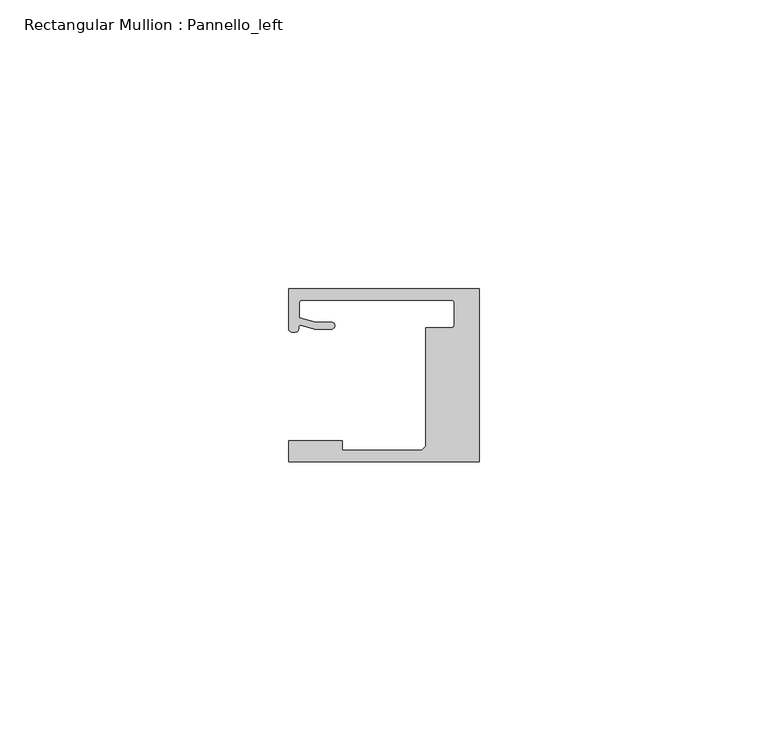
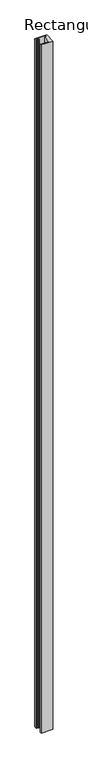
"""IFC4 building model written with IfcOpenShell, lengths in millimetres: member geometry, Rectangular Mullion : Pannello_left."""

from ifc_helpers import new_model, si_unit, frame, origin, place, context, project, spatial, polyline, circle_curve, source, transform, mapped, element, save
from ifc_brep_helpers import plane_surface, cylinder_surface, revolved_surface, extruded_surface, spline_curve, advanced_brep


def rectangular_mullion_pannello_left_dfdf7ad4(model_context):
    return source(origin(), model_context, "Body", "AdvancedBrep", [
        advanced_brep(
        [(-33.0, -15.0, 0.0), (0.0, -15.0, 0.0), (0.0, 15.0, 0.0), (-33.0000135, 15.0, 0.0), (-33.0000135, 8.0000472, 0.0), (-30.9223017, 8.6490241, 0.0), (-28.4999305, 7.9999523, 0.0), (-25.59998, 7.9999523, 0.0), (-25.59998, 9.1999523, 0.0), (-28.3419477, 9.1999523, 0.0), (-31.19998, 9.9657591, 0.0), (-31.19998, 12.50001, 0.0), (-30.69998, 13.00001, 0.0), (-4.7999726, 13.00001, 0.0), (-4.2999726, 12.50001, 0.0), (-4.2999726, 8.7500595, 0.0), (-4.7999726, 8.2500595, 0.0), (-9.2999726, 8.2500595, 0.0), (-9.2999726, -12.2999849, 0.0), (-10.0000103, -13.0000004, 0.0), (-23.700041, -13.0000004, 0.0), (-23.700041, -11.3000004, 0.0), (-33.0, -11.3000004, 0.0), (-33.0, -15.0, -2046.9999865), (-33.0, -11.3000004, -2046.9999865), (-23.700041, -11.3000004, -2046.9999865), (-23.700041, -13.0000004, -2046.9999865), (-10.0000103, -13.0000004, -2046.9999865), (-9.2999726, -12.2999849, -2046.9999865), (-9.2999726, 8.2500595, -2046.9999865), (-4.7999726, 8.2500595, -2046.9999865), (-4.2999726, 8.7500595, -2046.9999865), (-4.2999726, 12.50001, -2046.9999865), (-4.7999726, 13.00001, -2046.9999865), (-30.69998, 13.00001, -2046.9999865), (-31.19998, 12.50001, -2046.9999865), (-31.19998, 9.9657591, -2046.9999865), (-28.3419477, 9.1999523, -2046.9999865), (-25.59998, 9.1999523, -2046.9999865), (-25.59998, 7.9999523, -2046.9999865), (-28.4999305, 7.9999523, -2046.9999865), (-30.9223017, 8.6490241, -2046.9999865), (-33.0000135, 8.0000472, -2046.9999865), (-33.0000135, 15.0, -2046.9999865), (0.0, 15.0, -2046.9999865), (0.0, -15.0, -2046.9999865)],
        [
            (0, 1),
            (1, 2),
            (2, 3),
            (3, 4),
            (4, 5, spline_curve(3, [(-33.0000135, 8.0000472, 0.0), (-33.0000135, 7.457047519, 0.0), (-32.262327879, 7.456527435, 0.0), (-31.357433266, 7.563996614, 0.0), (-31.305645054, 7.690065204, 0.0), (-31.298563602, 8.366228555, 0.0), (-31.312054066, 8.717747958, 0.0), (-30.9223017, 8.6490241, 0.0)], [4, 2, 2, 4], [0.0, 0.0027053965905959043, 0.0058611956533709, 0.007702013405570312])),
            (5, 6),
            (6, 7),
            (7, 8, circle_curve(frame((-25.59998, 8.5999523, 0.0), z_axis=(0.0, 0.0, 1.0), x_axis=(0.0, 1.0, 0.0)), 0.6)),
            (8, 9),
            (9, 10),
            (10, 11),
            (11, 12, circle_curve(frame((-30.69998, 12.50001, 0.0), z_axis=(0.0, 0.0, -1.0), x_axis=(0.0, 1.0, 0.0)), 0.5)),
            (12, 13),
            (13, 14, circle_curve(frame((-4.7999726, 12.50001, 0.0), z_axis=(0.0, 0.0, -1.0), x_axis=(1.0, 0.0, 0.0)), 0.5)),
            (14, 15),
            (15, 16, circle_curve(frame((-4.7999726, 8.7500595, 0.0), z_axis=(0.0, 0.0, -1.0), x_axis=(0.0, -1.0, 0.0)), 0.5)),
            (16, 17),
            (17, 18),
            (18, 19),
            (19, 20),
            (20, 21),
            (21, 22),
            (22, 0),
            (23, 24),
            (24, 25),
            (25, 26),
            (26, 27),
            (27, 28),
            (28, 29),
            (29, 30),
            (30, 31, circle_curve(frame((-4.7999726, 8.7500595, -2046.9999865), z_axis=(0.0, 0.0, 1.0), x_axis=(0.0, -1.0, 0.0)), 0.5)),
            (31, 32),
            (32, 33, circle_curve(frame((-4.7999726, 12.50001, -2046.9999865), z_axis=(0.0, 0.0, 1.0), x_axis=(1.0, 0.0, 0.0)), 0.5)),
            (33, 34),
            (34, 35, circle_curve(frame((-30.69998, 12.50001, -2046.9999865), z_axis=(0.0, 0.0, 1.0), x_axis=(0.0, 1.0, 0.0)), 0.5)),
            (35, 36),
            (36, 37),
            (37, 38),
            (38, 39, circle_curve(frame((-25.59998, 8.5999523, -2046.9999865), z_axis=(0.0, 0.0, -1.0), x_axis=(0.0, 1.0, 0.0)), 0.6)),
            (39, 40),
            (40, 41),
            (41, 42, spline_curve(3, [(-30.9223017, 8.6490241, -2046.9999865), (-31.312054066, 8.717747958, -2046.9999865), (-31.298563602, 8.366228555, -2046.9999865), (-31.305645054, 7.690065204, -2046.9999865), (-31.357433266, 7.563996614, -2046.9999865), (-32.262327879, 7.456527435, -2046.9999865), (-33.0000135, 7.457047519, -2046.9999865), (-33.0000135, 8.0000472, -2046.9999865)], [4, 2, 2, 4], [0.0, 0.001840817752199412, 0.004996616814974408, 0.007702013405570312])),
            (42, 43),
            (43, 44),
            (44, 45),
            (45, 23),
            (0, 23),
            (45, 1),
            (44, 2),
            (43, 3),
            (42, 4),
            (41, 5),
            (40, 6),
            (39, 7),
            (38, 8),
            (37, 9),
            (36, 10),
            (35, 11),
            (34, 12),
            (33, 13),
            (32, 14),
            (31, 15),
            (30, 16),
            (29, 17),
            (28, 18),
            (27, 19),
            (26, 20),
            (25, 21),
            (24, 22),
        ],
        [
            plane_surface(frame((0.0, -36.2491502, 0.0), z_axis=(0.0, 0.0, 1.0), x_axis=(-1.0, 0.0, 0.0))),
            plane_surface(frame((0.0, -36.2491502, -2046.9999865), z_axis=(0.0, 0.0, -1.0), x_axis=(-1.0, 0.0, 0.0))),
            plane_surface(frame((-33.0, -15.0, 0.0), z_axis=(0.0, -1.0, 0.0), x_axis=(0.0, 0.0, -1.0))),
            plane_surface(frame((0.0, -15.0, 0.0), z_axis=(1.0, 0.0, 0.0), x_axis=(0.0, 0.0, -1.0))),
            plane_surface(frame((0.0, 15.0, 0.0), z_axis=(0.0, 1.0, 0.0), x_axis=(0.0, 0.0, -1.0))),
            plane_surface(frame((-33.0000135, 15.0, 0.0), z_axis=(-1.0, 0.0, 0.0), x_axis=(0.0, 0.0, -1.0))),
            extruded_surface(spline_curve(3, [(-33.0000135, 8.0000472, -2046.9999865), (-33.0000135, 7.457047519, -2046.9999865), (-32.262327879, 7.456527435, -2046.9999865), (-31.357433266, 7.563996614, -2046.9999865), (-31.305645054, 7.690065204, -2046.9999865), (-31.298563602, 8.366228555, -2046.9999865), (-31.312054066, 8.717747958, -2046.9999865), (-30.9223017, 8.6490241, -2046.9999865)], [4, 2, 2, 4], [0.0, 0.0027053965905959043, 0.0058611956533709, 0.007702013405570312]), (0.0, 0.0, 2046.9999865), 2046.9999865),
            plane_surface(frame((-30.9223017, 8.6490241, 0.0), z_axis=(-0.25881883200192934, -0.9659258833891746, 0.0), x_axis=(0.0, 0.0, -1.0))),
            plane_surface(frame((-28.4999305, 7.9999523, 0.0), z_axis=(0.0, -1.0, 0.0), x_axis=(0.0, 0.0, -1.0))),
            cylinder_surface(frame((-25.59998, 8.5999523, 0.0), z_axis=(0.0, 0.0, 1.0), x_axis=(0.0, 1.0, 0.0)), 0.6),
            plane_surface(frame((-25.59998, 9.1999523, 0.0), z_axis=(0.0, 1.0, 0.0), x_axis=(0.0, 0.0, -1.0))),
            plane_surface(frame((-28.3419477, 9.1999523, 0.0), z_axis=(0.25881883204288636, 0.9659258833782002, 0.0), x_axis=(0.0, 0.0, -1.0))),
            plane_surface(frame((-31.19998, 9.9657591, 0.0), z_axis=(1.0, 0.0, 0.0), x_axis=(0.0, 0.0, -1.0))),
            revolved_surface(polyline([(-30.69998, 13.00001, -2046.9999865), (-30.69998, 13.00001, 0.0)]), (-30.69998, 12.50001, 0.0), (0.0, 0.0, -1.0)),
            plane_surface(frame((-30.69998, 13.00001, 0.0), z_axis=(0.0, -1.0, 0.0), x_axis=(0.0, 0.0, -1.0))),
            revolved_surface(polyline([(-4.2999726, 12.50001, -2046.9999865), (-4.2999726, 12.50001, 0.0)]), (-4.7999726, 12.50001, 0.0), (0.0, 0.0, -1.0)),
            plane_surface(frame((-4.2999726, 12.50001, 0.0), z_axis=(-1.0, 0.0, 0.0), x_axis=(0.0, 0.0, -1.0))),
            revolved_surface(polyline([(-4.7999726, 8.2500595, -2046.9999865), (-4.7999726, 8.2500595, 0.0)]), (-4.7999726, 8.7500595, 0.0), (0.0, 0.0, -1.0)),
            plane_surface(frame((-4.7999726, 8.2500595, 0.0), z_axis=(0.0, 1.0, 0.0), x_axis=(0.0, 0.0, -1.0))),
            plane_surface(frame((-9.2999726, 8.2500595, 0.0), z_axis=(-1.0, 0.0, 0.0), x_axis=(0.0, 0.0, -1.0))),
            plane_surface(frame((-9.2999726, -12.2999849, 0.0), z_axis=(-0.7070955486277984, 0.7071180135668678, 0.0), x_axis=(0.0, 0.0, -1.0))),
            plane_surface(frame((-10.0000103, -13.0000004, 0.0), z_axis=(0.0, 1.0, 0.0), x_axis=(0.0, 0.0, -1.0))),
            plane_surface(frame((-23.700041, -13.0000004, 0.0), z_axis=(1.0, 0.0, 0.0), x_axis=(0.0, 0.0, -1.0))),
            plane_surface(frame((-23.700041, -11.3000004, 0.0), z_axis=(0.0, 1.0, 0.0), x_axis=(0.0, 0.0, -1.0))),
            plane_surface(frame((-33.0, -11.3000004, 0.0), z_axis=(-1.0, 0.0, 0.0), x_axis=(0.0, 0.0, -1.0))),
        ],
        [
            (0, [[1, 2, 3, 4, 5, 6, 7, 8, 9, 10, 11, 12, 13, 14, 15, 16, 17, 18, 19, 20, 21, 22, 23]]),
            (1, [[24, 25, 26, 27, 28, 29, 30, 31, 32, 33, 34, 35, 36, 37, 38, 39, 40, 41, 42, 43, 44, 45, 46]]),
            (2, [[-1, 47, -46, 48]]),
            (3, [[-2, -48, -45, 49]]),
            (4, [[-3, -49, -44, 50]]),
            (5, [[-4, -50, -43, 51]]),
            (6, [[-5, -51, -42, 52]]),
            (7, [[-6, -52, -41, 53]]),
            (8, [[-7, -53, -40, 54]]),
            (9, [[-8, -54, -39, 55]]),
            (10, [[-9, -55, -38, 56]]),
            (11, [[-10, -56, -37, 57]]),
            (12, [[-11, -57, -36, 58]]),
            (13, [[-12, -58, -35, 59]]),
            (14, [[-13, -59, -34, 60]]),
            (15, [[-14, -60, -33, 61]]),
            (16, [[-15, -61, -32, 62]]),
            (17, [[-16, -62, -31, 63]]),
            (18, [[-17, -63, -30, 64]]),
            (19, [[-18, -64, -29, 65]]),
            (20, [[-19, -65, -28, 66]]),
            (21, [[-20, -66, -27, 67]]),
            (22, [[-21, -67, -26, 68]]),
            (23, [[-22, -68, -25, 69]]),
            (24, [[-23, -69, -24, -47]]),
        ],
    ),
    ])


if __name__ == "__main__":
    model = new_model("IFC4")
    model_context = context("Model", 3, world=origin())
    ifc_project = project(units=[si_unit("LENGTHUNIT", "METRE", prefix="MILLI")], contexts=[model_context])
    site = spatial("IfcSite", under=ifc_project)
    building = spatial("IfcBuilding", under=site)
    placement = place(None, origin())
    rectangular_mullion_pannello_left_shape = rectangular_mullion_pannello_left_dfdf7ad4(model_context)
    element("IfcMember", 1, ObjectType="Rectangular Mullion : Pannello_left", at=placement, inside=building, context=model_context, shape_type="MappedRepresentation", body=[
        mapped(rectangular_mullion_pannello_left_shape, transform((0.0, 0.0, 0.0), x_axis=(1.0, 0.0, 0.0), y_axis=(0.0, 1.0, 0.0), z_axis=(0.0, 0.0, 1.0))),
    ])
    save(model, "model.ifc")

# Revit data of these elements
# Type "Rectangular Mullion : Pannello_left"
#   built-in parameter 1007322 = 0.0984252 (stored number, unit not read)
#   built-in parameter 1007320 = 0.0305117 (stored number, unit not read)
